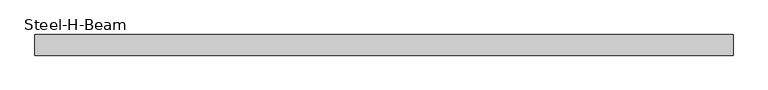
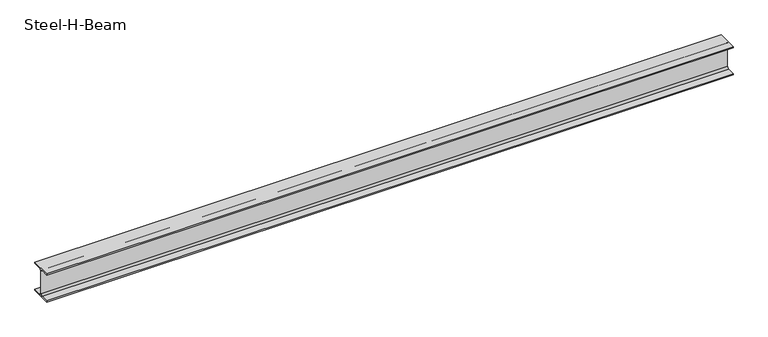
"""IFC4 building model written with IfcOpenShell, lengths in millimetres: beam geometry, Steel-H-Beam : BM121_H-294×200x8x12."""

import ifcopenshell
import ifcopenshell.guid

model = None  # the IFC model being written
_history = None  # IfcOwnerHistory: only IFC2X3 demands one
_inside = {}  # id of a spatial element -> (the spatial element, [elements in it])
_under = {}  # id of a project, library or spatial element -> (it, [spatial elements below it])
_declared = {}  # id of a project -> (the project, [libraries it declares])
_typed = {}  # id of a type object -> (the type object, [elements of that type])
_made_of = {}  # id of a material, layer set ... -> (it, [elements and type objects made of it])


def new_model(schema):
    """Start an empty IFC model of exactly this schema.

    Asked for "IFC4X3", IfcOpenShell would pick the latest addendum, in which some entities
    have other attributes; the version numbers below select the first issue.
    IFC2X3 requires an IfcOwnerHistory on every rooted entity: one is made here for all.
    """
    global model, _history
    if schema == "IFC4X3":
        model = ifcopenshell.file(schema_version=(4, 3, 0, 0))
    else:
        model = ifcopenshell.file(schema=schema)
    _inside.clear()
    _under.clear()
    _declared.clear()
    _typed.clear()
    _made_of.clear()
    _history = None
    if model.schema == "IFC2X3":
        org = make("IfcOrganization", Name="unknown")
        user = make(
            "IfcPersonAndOrganization",
            ThePerson=make("IfcPerson", FamilyName="unknown"),
            TheOrganization=org,
        )
        app = make(
            "IfcApplication",
            ApplicationDeveloper=org,
            Version="unknown",
            ApplicationFullName="unknown",
            ApplicationIdentifier="unknown",
        )
        _history = make(
            "IfcOwnerHistory",
            OwningUser=user,
            OwningApplication=app,
            ChangeAction="ADDED",
            CreationDate=0,
        )
    return model


def make(cls, **values):
    """One entity of the class cls with the attributes given. An attribute that is None is left unset."""
    return model.create_entity(
        cls, **{name: value for name, value in values.items() if value is not None}
    )


def rooted(cls, **values):
    """An entity with a GlobalId (a new one), such as an element, a storey or a relation."""
    return make(cls, GlobalId=ifcopenshell.guid.new(), OwnerHistory=_history, **values)


def si_unit(unit_type, name, prefix=None):
    """IfcSIUnit, for example si_unit("LENGTHUNIT", "METRE", prefix="MILLI")."""
    return make("IfcSIUnit", UnitType=unit_type, Prefix=prefix, Name=name)


def assignment(units):
    """IfcUnitAssignment: the units of a project."""
    return None if units is None else make("IfcUnitAssignment", Units=units)


def point(xyz):
    """IfcCartesianPoint."""
    return None if xyz is None else make("IfcCartesianPoint", Coordinates=xyz)


def direction(xyz):
    """IfcDirection."""
    return None if xyz is None else make("IfcDirection", DirectionRatios=xyz)


def frame(location, z_axis=None, x_axis=None):
    """IfcAxis2Placement3D, a coordinate frame: its origin and axes. An axis left out is left unset."""
    return make(
        "IfcAxis2Placement3D",
        Location=point(location),
        Axis=direction(z_axis),
        RefDirection=direction(x_axis),
    )


def frame_2d(location, x_axis=None):
    """IfcAxis2Placement2D, a coordinate frame in the plane: its origin and x axis."""
    return make(
        "IfcAxis2Placement2D", Location=point(location), RefDirection=direction(x_axis)
    )


def origin():
    """The frame at (0, 0, 0) with its axes left unset."""
    return frame((0.0, 0.0, 0.0))


def place(relative_to, where):
    """IfcLocalPlacement: puts the frame where relative to a parent placement (None: the world)."""
    return make(
        "IfcLocalPlacement", PlacementRelTo=relative_to, RelativePlacement=where
    )


def context(
    kind, dimensions, precision=None, world=None, true_north=None, identifier=None
):
    """IfcGeometricRepresentationContext, for example the 3D "Model" context."""
    return make(
        "IfcGeometricRepresentationContext",
        ContextIdentifier=identifier,
        ContextType=kind,
        CoordinateSpaceDimension=dimensions,
        Precision=precision,
        WorldCoordinateSystem=world,
        TrueNorth=true_north,
    )


def project(units=None, contexts=None):
    """IfcProject with its units and contexts."""
    return rooted(
        "IfcProject",
        Name="project",
        RepresentationContexts=contexts,
        UnitsInContext=assignment(units),
    )


def spatial(cls, under=None, at=None, **own):
    """A site, building, storey or space (cls), placed at a placement, below another one or the project."""
    s = rooted(cls, ObjectPlacement=at, **own)
    if under is not None:
        _under.setdefault(under.id(), (under, []))[1].append(s)
    return s


def polyline(points):
    """IfcPolyline through the points."""
    return make("IfcPolyline", Points=[point(p) for p in points])


def circle_curve(where, radius):
    """IfcCircle in the frame where."""
    return make("IfcCircle", Position=where, Radius=radius)


def trimmed(basis, trim1, trim2, sense, master):
    """IfcTrimmedCurve: the piece of a basis curve between two trims."""
    return make(
        "IfcTrimmedCurve",
        BasisCurve=basis,
        Trim1=trim1,
        Trim2=trim2,
        SenseAgreement=sense,
        MasterRepresentation=master,
    )


def segment(curve, same_sense, transition):
    """IfcCompositeCurveSegment."""
    return make(
        "IfcCompositeCurveSegment",
        Transition=transition,
        SameSense=same_sense,
        ParentCurve=curve,
    )


def composite_curve(segments, self_intersect=None):
    """IfcCompositeCurve: segments joined end to end."""
    return make("IfcCompositeCurve", Segments=segments, SelfIntersect=self_intersect)


def outline(outer, holes=None, kind="AREA"):
    """IfcArbitraryClosedProfileDef: a profile drawn as a closed curve; with holes, ...WithVoids."""
    if holes is None:
        return make("IfcArbitraryClosedProfileDef", ProfileType=kind, OuterCurve=outer)
    return make(
        "IfcArbitraryProfileDefWithVoids",
        ProfileType=kind,
        OuterCurve=outer,
        InnerCurves=holes,
    )


def extrude(swept, where, along, depth):
    """IfcExtrudedAreaSolid: the profile swept, set in the frame where, extruded along a direction by depth."""
    return make(
        "IfcExtrudedAreaSolid",
        SweptArea=swept,
        Position=where,
        ExtrudedDirection=direction(along),
        Depth=depth,
    )


def shape(context_of_items, identifier, shape_type, items):
    """IfcShapeRepresentation: the items that make up one representation, for example the "Body"."""
    return make(
        "IfcShapeRepresentation",
        ContextOfItems=context_of_items,
        RepresentationIdentifier=identifier,
        RepresentationType=shape_type,
        Items=items,
    )


def source(mapping_origin, context_of_items, identifier, shape_type, items):
    """IfcRepresentationMap: a shape defined once, which mapped items show again and again."""
    return make(
        "IfcRepresentationMap",
        MappingOrigin=mapping_origin,
        MappedRepresentation=shape(context_of_items, identifier, shape_type, items),
    )


def transform(
    local_origin,
    x_axis=None,
    y_axis=None,
    z_axis=None,
    scale=None,
    scale2=None,
    scale3=None,
    uniform=True,
):
    """IfcCartesianTransformationOperator3D, or its non-uniform kind. x_axis, y_axis, z_axis: its Axis1, 2, 3."""
    if uniform:
        return make(
            "IfcCartesianTransformationOperator3D",
            Axis1=direction(x_axis),
            Axis2=direction(y_axis),
            LocalOrigin=point(local_origin),
            Scale=scale,
            Axis3=direction(z_axis),
        )
    return make(
        "IfcCartesianTransformationOperator3DnonUniform",
        Axis1=direction(x_axis),
        Axis2=direction(y_axis),
        LocalOrigin=point(local_origin),
        Scale=scale,
        Axis3=direction(z_axis),
        Scale2=scale2,
        Scale3=scale3,
    )


def mapped(mapping_source, mapping_target):
    """IfcMappedItem: shows the shape of a source again, moved by a transform."""
    return make(
        "IfcMappedItem", MappingSource=mapping_source, MappingTarget=mapping_target
    )


def made_of(thing, what):
    """Note that an element or type object is made of a material, layer set ...; save() writes the relation."""
    if what is not None:
        _made_of.setdefault(what.id(), (what, []))[1].append(thing)
    return thing


def element(
    cls,
    number,
    at=None,
    inside=None,
    cuts=None,
    type_object=None,
    material=None,
    context=None,
    identifier="Body",
    shape_type=None,
    held_by="IfcProductDefinitionShape",
    body=None,
    shapes=None,
    **own,
):
    """One element of the class cls, such as IfcWall. Its Tag is "e" and its number.

    at: its placement. inside: the storey or other place that contains it. cuts: it is an
    opening in that element (IfcRelVoidsElement). A single representation is given by context,
    identifier, shape_type and body (its items); several are given by shapes. held_by: the class
    of the entity that holds the representations. save() writes the other relations.
    """
    e = rooted(cls, Tag="e%d" % number, ObjectPlacement=at, **own)
    if body is not None:
        shapes = [shape(context, identifier, shape_type, body)]
    if shapes is not None:
        e.Representation = make(held_by, Representations=shapes)
    if inside is not None:
        _inside.setdefault(inside.id(), (inside, []))[1].append(e)
    if cuts is not None:
        rooted(
            "IfcRelVoidsElement", RelatingBuildingElement=cuts, RelatedOpeningElement=e
        )
    if type_object is not None:
        _typed.setdefault(type_object.id(), (type_object, []))[1].append(e)
    return made_of(e, material)


def aggregate(whole, parts):
    """IfcRelAggregates: a whole, such as a stair, and the parts it consists of."""
    return rooted("IfcRelAggregates", RelatingObject=whole, RelatedObjects=parts)


def save(model, path):
    """Write the relations noted so far, then the file.

    IfcRelAggregates (storeys below a building ...), IfcRelContainedInSpatialStructure (elements
    in a storey), IfcRelDefinesByType, IfcRelAssociatesMaterial and IfcRelDeclares: one each for
    every whole, place, type object, material and project.
    """
    for whole, parts in _under.values():
        aggregate(whole, parts)
    for where, things in _inside.values():
        rooted(
            "IfcRelContainedInSpatialStructure",
            RelatedElements=things,
            RelatingStructure=where,
        )
    for kind, things in _typed.values():
        rooted("IfcRelDefinesByType", RelatedObjects=things, RelatingType=kind)
    for what, things in _made_of.values():
        rooted("IfcRelAssociatesMaterial", RelatedObjects=things, RelatingMaterial=what)
    for by, libraries in _declared.values():
        rooted("IfcRelDeclares", RelatingContext=by, RelatedDefinitions=libraries)
    model.write(path)


def steel_h_beam_4d9bb108(model_context):
    return source(origin(), model_context, "Body", "SweptSolid", [
        extrude(outline(composite_curve([segment(polyline([(100.0, -135.0), (100.0, -147.0), (-100.0, -147.0), (-100.0, -135.0), (-22.0, -135.0)]), True, "CONTINUOUS"), segment(trimmed(circle_curve(frame_2d((-22.0, -117.0)), 18.0), [point((-22.0, -135.0))], [point((-4.0, -117.0))], True, "CARTESIAN"), True, "CONTINUOUS"), segment(polyline([(-4.0, -117.0), (-4.0, 117.0)]), True, "CONTINUOUS"), segment(trimmed(circle_curve(frame_2d((-22.0, 117.0)), 18.0), [point((-4.0, 117.0))], [point((-22.0, 135.0))], True, "CARTESIAN"), True, "CONTINUOUS"), segment(polyline([(-22.0, 135.0), (-100.0, 135.0), (-100.0, 147.0), (100.0, 147.0), (100.0, 135.0), (22.0, 135.0)]), True, "CONTINUOUS"), segment(trimmed(circle_curve(frame_2d((22.0, 117.0)), 18.0), [point((22.0, 135.0))], [point((4.0, 117.0))], True, "CARTESIAN"), True, "CONTINUOUS"), segment(polyline([(4.0, 117.0), (4.0, -117.0)]), True, "CONTINUOUS"), segment(trimmed(circle_curve(frame_2d((22.0, -117.0)), 18.0), [point((4.0, -117.0))], [point((22.0, -135.0))], True, "CARTESIAN"), True, "CONTINUOUS"), segment(polyline([(22.0, -135.0), (100.0, -135.0)]), True, "CONTINUOUS")], self_intersect=False)), frame((-3390.0, 0.0, 0.0), z_axis=(1.0, 0.0, 0.0), x_axis=(0.0, 1.0, 0.0)), (0.0, 0.0, 1.0), 6780.0),
    ])


if __name__ == "__main__":
    model = new_model("IFC4")
    model_context = context("Model", 3, world=origin())
    ifc_project = project(units=[si_unit("LENGTHUNIT", "METRE", prefix="MILLI")], contexts=[model_context])
    site = spatial("IfcSite", under=ifc_project)
    building = spatial("IfcBuilding", under=site)
    placement = place(None, origin())
    steel_h_beam_shape = steel_h_beam_4d9bb108(model_context)
    element("IfcBeam", 1, ObjectType="Steel-H-Beam : BM121_H-294×200x8x12", at=placement, inside=building, context=model_context, shape_type="MappedRepresentation", body=[
        mapped(steel_h_beam_shape, transform((0.0, 0.0, 0.0), x_axis=(1.0, 0.0, 0.0), y_axis=(0.0, 1.0, 0.0), z_axis=(0.0, 0.0, 1.0))),
    ])
    save(model, "model.ifc")

# Revit data of these elements
# Type "Steel-H-Beam : BM121_H-294×200x8x12"
#   Surface Area = 1.3411 m²/m
#   Section Area = 72.3812 cm²
#   Mass per Unit Length = 56.8193 kg/m
#   Length [instance default] = 3000 mm
#   B = 200 mm
#   H = 294 mm
#   r = 18 mm
#   tw = 8 mm
#   tf = 12 mm
#   hec_material4 [instance default] = none
#   hec_material3 [instance default] = none
#   hec_material2 [instance default] = none
#   hec_material1 [instance default] = none
#   Structural Material [instance default] = Steel, 45-345
#   Assembly Code = ""
# Element 1 (IfcBeam, "Steel-H-Beam : BM121_H-294×200x8x12")
#   hec_material3 = F01AC000-00002_Building/Shelter Fire Proofing Work_Intumescent Coating Type_1 hr. rating (UL 1709))
#   hec_material2 = S01AA010-00002_Main Steel Structure Fabrication Work_Shelter/Building_Steel Painting/Coating_for Fireproofed Steel Surface, Surface Preparation & Primer Coat
#   hec_material1 = S03AA028-00001_Main Steel Structure Erection Work_Shelter/Building_Medium Steel
#   Structural Material = S01AA002-00001_Main Steel Structure Fabrication Work_Shelter/Building_Medium Steel - Standard
#   Materials on its faces: "S01AA002-00001_Main Steel Structure Fabrication Work_Shelter/Building_Medium Steel - Standard"
# Materials
#   "Steel, 45-345": class "Metal", colour RGB 189 187 185, transparency 0, Description = "Steel 345 MPa", Cost = 0
#   "S01AA002-00001_Main Steel Structure Fabrication Work_Shelter/Building_Medium Steel - Standard": class "Metal", colour RGB 120 120 120, transparency 0, Comments = "(90KG/M>Weight≥30KG/M)", Description = "Structural steel 50ksi", W00) Work Master Code = "S01AA002-0001", W01) Work Master_Lv1 = "Main Steel Structure Fabrication Work", W02) Work Master_Lv2 = "Shelter/Building", W03) Work Master_Spec.1 = "Medium Steel - Standard (90KG/M>Weight≥30KG/M)", Cost = 0
#   "F01AC000-00002_Building/Shelter Fire Proofing Work_Intumescent Coating Type_1 hr. rating (UL 1709))": class "Metal", colour RGB 255 128 128, transparency 0, Description = "Paint finished steel", W00) Work Master Code = "F01AC000-00002", W01) Work Master_Lv1 = "Building/Shelter Fire Proofing Work", W02) Work Master_Lv2 = "Intumescent Coating Type", W03) Work Master_Spec.1 = "1 hr. rating (UL 1709)", Cost = 0
#   "S01AA010-00002_Main Steel Structure Fabrication Work_Shelter/Building_Steel Painting/Coating_for Fireproofed Steel Surface, Surface Preparation & Primer Coat": class "Metal", colour RGB 120 120 120, transparency 0, Description = "Paint finished steel", W00) Work Master Code = "SS01AA010-00002", W01) Work Master_Lv1 = "Main Steel Structure Fabrication Work", W02) Work Master_Lv2 = "Shelter/Building", W03) Work Master_Spec.1 = "Steel Painting/Coating", W04) Work Master_Spec.2 = "for Fireproofed Steel Surface, Surface Preparation & Primer Coat", Cost = 0
#   "S03AA028-00001_Main Steel Structure Erection Work_Shelter/Building_Medium Steel": class "Metal", colour RGB 120 120 120, transparency 0, Comments = "(90KG/M>Weight≥30KG/M)", Description = "Structural steel 50ksi", W00) Work Master Code = "S03AA028-0001", W01) Work Master_Lv1 = "Main Steel Structure Erection Work", W02) Work Master_Lv2 = "Shelter/Building", W03) Work Master_Spec.1 = "Medium Steel (90KG/M>Weight≥30KG/M)", Cost = 0
